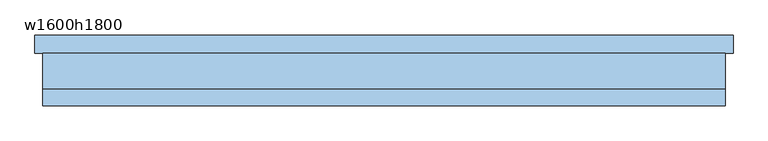
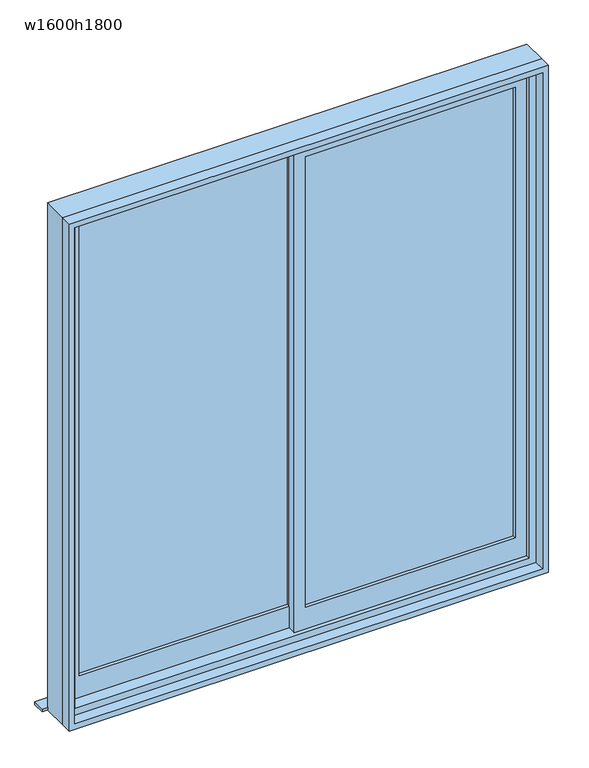
"""IFC4 building model written with IfcOpenShell, lengths in millimetres: window geometry, 引違い掃出窓_2枚 : w1600h1800."""

from ifc_helpers import new_model, si_unit, frame, origin, place, context, project, spatial, polyline, outline, extrude, source, transform, mapped, element, save


def w1600h1800_bd36f67d(model_context):
    return source(origin(), model_context, "Body", "SweptSolid", [
        extrude(outline(polyline([(-20.0, 12.5), (-760.0, 12.5), (-760.0, 17.5), (-20.0, 17.5), (-20.0, 12.5)])), frame((0.0, 0.0, 280.0), z_axis=(0.0, 0.0, 1.0), x_axis=(1.0, 0.0, 0.0)), (0.0, 0.0, 1.0), 1680.0),
        extrude(outline(polyline([(760.0, -17.5), (20.0, -17.5), (20.0, -12.5), (760.0, -12.5), (760.0, -17.5)])), frame((0.0, 0.0, 280.0), z_axis=(0.0, 0.0, 1.0), x_axis=(1.0, 0.0, 0.0)), (0.0, 0.0, 1.0), 1680.0),
        extrude(outline(polyline([(2000.0, -20.0), (200.0, -20.0), (200.0, 800.0), (2000.0, 800.0), (2000.0, -20.0)]), holes=[polyline([(280.0, 760.0), (280.0, 20.0), (1960.0, 20.0), (1960.0, 760.0), (280.0, 760.0)])]), frame((0.0, -30.0, 0.0), z_axis=(0.0, 1.0, 0.0), x_axis=(0.0, 0.0, 1.0)), (0.0, 0.0, 1.0), 30.0),
        extrude(outline(polyline([(2000.0, -800.0), (200.0, -800.0), (200.0, 20.0), (2000.0, 20.0), (2000.0, -800.0)]), holes=[polyline([(280.0, -20.0), (280.0, -760.0), (1960.0, -760.0), (1960.0, -20.0), (280.0, -20.0)])]), frame((0.0, 0.0, 0.0), z_axis=(0.0, 1.0, 0.0), x_axis=(0.0, 0.0, 1.0)), (0.0, 0.0, 1.0), 30.0),
        extrude(outline(polyline([(865.0, 90.0), (865.0, 45.0), (-865.0, 45.0), (-865.0, 90.0), (865.0, 90.0)])), frame((0.0, 0.0, 155.0), z_axis=(0.0, 0.0, 1.0), x_axis=(1.0, 0.0, 0.0)), (0.0, 0.0, 1.0), 10.0),
        extrude(outline(polyline([(2045.0, 845.0), (2045.0, -845.0), (155.0, -845.0), (155.0, 845.0), (2045.0, 845.0)]), holes=[polyline([(175.0, -825.0), (2025.0, -825.0), (2025.0, 825.0), (175.0, 825.0), (175.0, -825.0)])]), frame((0.0, -85.0, 0.0), z_axis=(0.0, 1.0, 0.0), x_axis=(0.0, 0.0, 1.0)), (0.0, 0.0, 1.0), 40.0),
        extrude(outline(polyline([(2045.0, -845.0), (155.0, -845.0), (155.0, 845.0), (2045.0, 845.0), (2045.0, -845.0)]), holes=[polyline([(2000.0, 800.0), (200.0, 800.0), (200.0, -800.0), (2000.0, -800.0), (2000.0, 800.0)])]), frame((0.0, -45.0, 0.0), z_axis=(0.0, 1.0, 0.0), x_axis=(0.0, 0.0, 1.0)), (0.0, 0.0, 1.0), 90.0),
    ])


if __name__ == "__main__":
    model = new_model("IFC4")
    model_context = context("Model", 3, world=origin())
    ifc_project = project(units=[si_unit("LENGTHUNIT", "METRE", prefix="MILLI")], contexts=[model_context])
    site = spatial("IfcSite", under=ifc_project)
    building = spatial("IfcBuilding", under=site)
    placement = place(None, origin())
    w1600h1800_shape = w1600h1800_bd36f67d(model_context)
    element("IfcWindow", 1, ObjectType="引違い掃出窓_2枚 : w1600h1800", at=placement, inside=building, context=model_context, shape_type="MappedRepresentation", body=[
        mapped(w1600h1800_shape, transform((0.0, 0.0, 0.0), x_axis=(1.0, 0.0, 0.0), y_axis=(0.0, 1.0, 0.0), z_axis=(0.0, 0.0, 1.0))),
    ])
    save(model, "model.ifc")

# Revit data of these elements
# Type "引違い掃出窓_2枚 : w1600h1800"
#   Construction Type Id = "GSP4R"
#   Analytic Construction = "1/8 インチ ピルキントン一重ガラス"
#   Type Mark = "67"
#   Operation = "ダブル パネル縦"
#   Keynote = "08520.R1"
#   Visual Light Transmittance = 0.9
#   Solar Heat Gain Coefficient = 0.86
#   Heat Transfer Coefficient (U) = 6.7069 W/(m²·K)
#   Height = 1800 mm
#   既定の腰高 = 200 mm
#   Width = 1600 mm
#   額縁見附 = 20 mm
#   額縁ちり = 10 mm
#   サッシ見附 = 45 mm
#   サッシの幅 = 90 mm
#   サッシ額縁 [instance default] = none
#   サッシ本体 [instance default] = none
#   サッシガラス [instance default] = ガラス - 透明
#   Manufacturer = ""
#   Wall Closure = (empty or 0)
#   Model = ""
#   Type Comments = ""
#   Assembly Code = ""
# Element 1 (IfcWindow, "引違い掃出窓_2枚 : w1600h1800")
#   Materials on its faces: "ガラス - 透明"
# Materials
#   "ガラス - 透明": class "ガラス", colour RGB 0 128 192, transparency 0.9, Cost = 0
